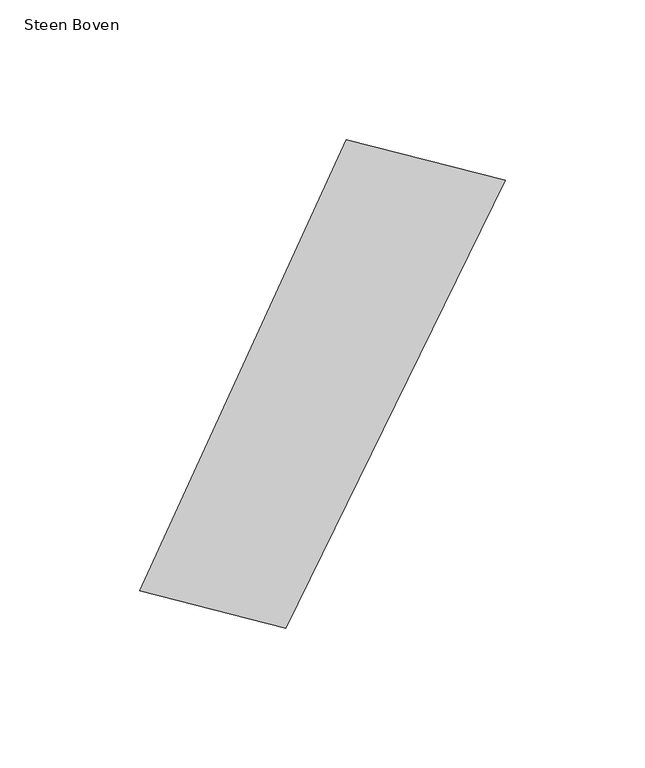
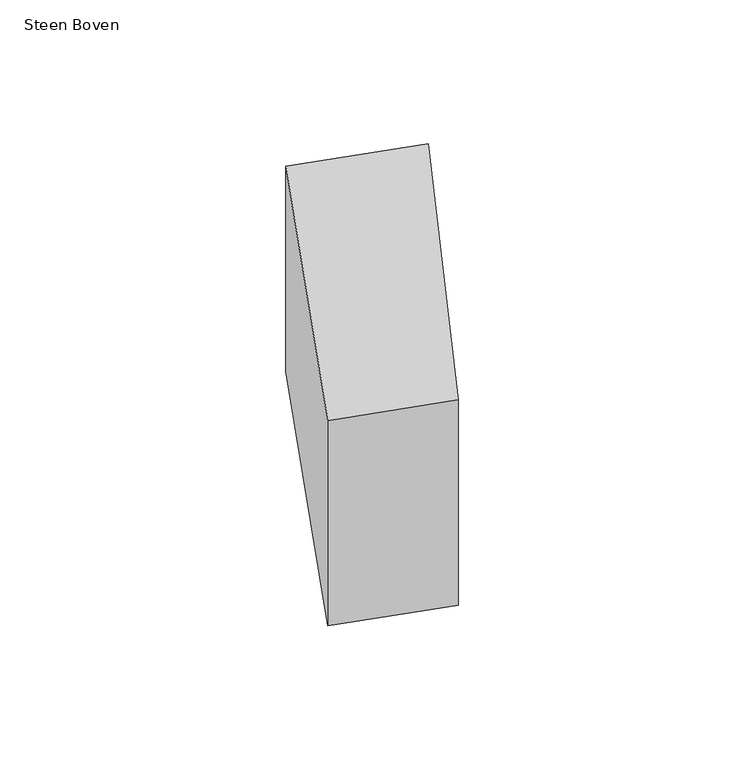
"""IFC4 building model written with IfcOpenShell, lengths in millimetres: proxy geometry, 00_GMA_steen_versie_4 : Steen Boven."""

from ifc_helpers import new_model, si_unit, origin, origin_with_axes, place, context, project, spatial, polyline, outline, extrude, source, transform, mapped, element, save


def steen_boven_01e32946(model_context):
    return source(origin(), model_context, "Body", "SweptSolid", [
        extrude(outline(polyline([(141.1704134, 152.36343), (62.4529027, -8.187695), (10.0350866, 5.3211774), (84.0648392, 167.0564768), (141.1704134, 152.36343)])), origin_with_axes(), (0.0, 0.0, 1.0), 100.0),
    ])


if __name__ == "__main__":
    model = new_model("IFC4")
    model_context = context("Model", 3, world=origin())
    ifc_project = project(units=[si_unit("LENGTHUNIT", "METRE", prefix="MILLI")], contexts=[model_context])
    site = spatial("IfcSite", under=ifc_project)
    building = spatial("IfcBuilding", under=site)
    placement = place(None, origin())
    steen_boven_shape = steen_boven_01e32946(model_context)
    element("IfcBuildingElementProxy", 1, Name="00_GMA_steen_versie_4 : Steen Boven", ObjectType="00_GMA_steen_versie_4 : Steen Boven", at=placement, inside=building, context=model_context, shape_type="MappedRepresentation", body=[
        mapped(steen_boven_shape, transform((0.0, 0.0, 0.0), x_axis=(1.0, 0.0, 0.0), y_axis=(0.0, 1.0, 0.0), z_axis=(0.0, 0.0, 1.0))),
    ])
    save(model, "model.ifc")

# Revit data of these elements
# Type "00_GMA_steen_versie_4 : Steen Boven"
#   StootVoegHalfBoven [instance default] = 5 mm
#   StootVoegHalf [instance default] = 5 mm
#   StootVoegBreedteOnder = 10 mm
#   StootVoegBreedteBoven = 10 mm
#   Steendikte = 100 mm
#   LintVoegOnderHalf = 5 mm
#   LintVoegOnder = 10 mm
#   LintVoegBovenHalf = 0 mm
#   LintVoegBoven = 0 mm
#   materiaal = none
#   MateriaalVoeg = none
#   Default Elevation = 0
